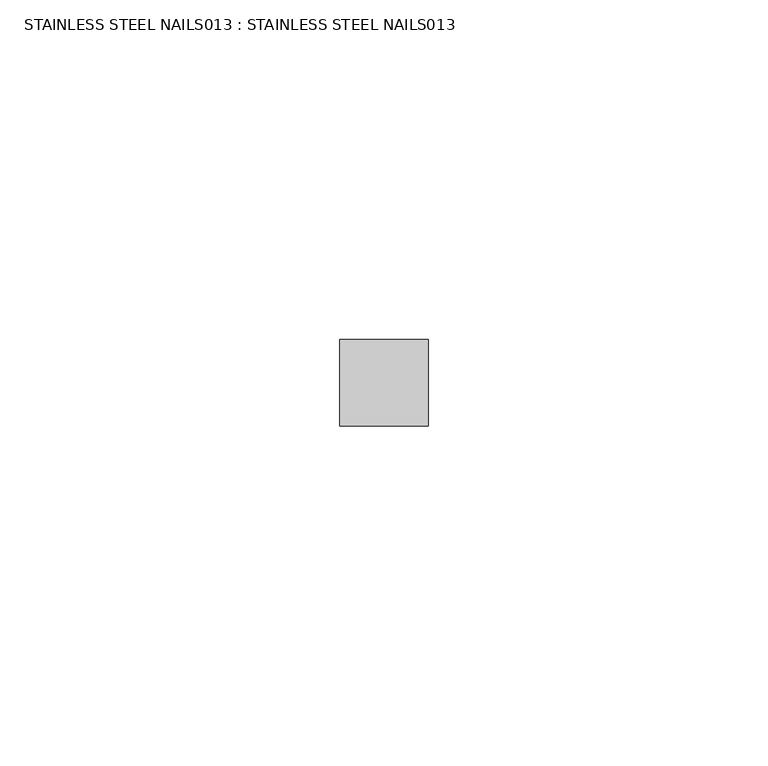
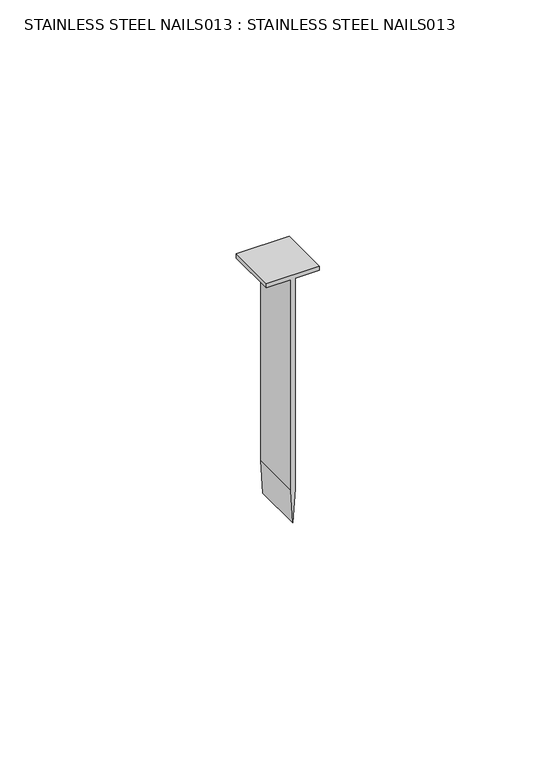
"""IFC4 building model written with IfcOpenShell, lengths in millimetres: proxy geometry, STAINLESS STEEL NAILS013 : STAINLESS STEEL NAILS013."""

from ifc_helpers import new_model, si_unit, frame, origin, place, context, project, spatial, polyline, outline, extrude, source, transform, mapped, element, save


def stainless_steel_nails013_stainless_steel_nails013_b095092e(model_context):
    return source(origin(), model_context, "Body", "SweptSolid", [
        extrude(outline(polyline([(40259.5998489, -4931.7136341), (40259.5998489, -4925.7560415), (40205.2729558, -4925.7560415), (40196.6073666, -4925.2144421), (40205.2729558, -4924.6728428), (40259.5998489, -4924.6728428), (40259.5998489, -4918.7152502), (40260.6830476, -4918.7152502), (40260.6830476, -4931.7136341), (40259.5998489, -4931.7136341)])), frame((0.0, -1065.5906573, 0.0), z_axis=(0.0, 1.0, 0.0), x_axis=(0.0, 0.0, 1.0)), (0.0, 0.0, 1.0), 12.7),
    ])


if __name__ == "__main__":
    model = new_model("IFC4")
    model_context = context("Model", 3, world=origin())
    ifc_project = project(units=[si_unit("LENGTHUNIT", "METRE", prefix="MILLI")], contexts=[model_context])
    site = spatial("IfcSite", under=ifc_project)
    building = spatial("IfcBuilding", under=site)
    placement = place(None, origin())
    stainless_steel_nails013_stainless_steel_nails013_shape = stainless_steel_nails013_stainless_steel_nails013_b095092e(model_context)
    element("IfcBuildingElementProxy", 1, Name="STAINLESS STEEL NAILS013 : STAINLESS STEEL NAILS013", ObjectType="STAINLESS STEEL NAILS013 : STAINLESS STEEL NAILS013", at=placement, inside=building, context=model_context, shape_type="MappedRepresentation", body=[
        mapped(stainless_steel_nails013_stainless_steel_nails013_shape, transform((0.0, 0.0, 0.0), x_axis=(1.0, 0.0, 0.0), y_axis=(0.0, 1.0, 0.0), z_axis=(0.0, 0.0, 1.0))),
    ])
    save(model, "model.ifc")

# Revit data of these elements
# Type "STAINLESS STEEL NAILS013 : STAINLESS STEEL NAILS013"
#   NameOverride = "STAINLESS STEEL NAILS013"
# Element 1 (IfcBuildingElementProxy, "STAINLESS STEEL NAILS013 : STAINLESS STEEL NAILS013")
#   Materials on its faces: "1 3/4\" STAINLESS STEEL RINGSHANK 5D COMMON NAILS @ 4\" (101.6MM) O.C. FIRESTONE PROVIDED MAX., 1/2\" STAGGERED"
# Materials
#   "1 3/4\" STAINLESS STEEL RINGSHANK 5D COMMON NAILS @ 4\" (101.6MM) O.C. FIRESTONE PROVIDED MAX., 1/2\" STAGGERED": class "Unassigned", colour RGB 255 255 255, transparency 0
